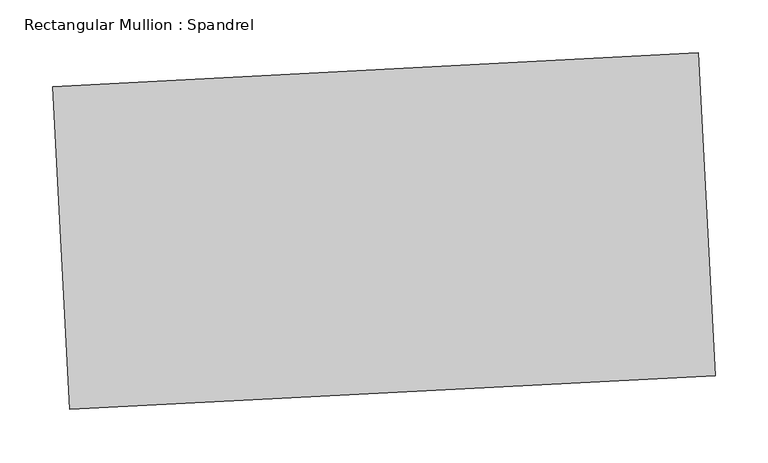
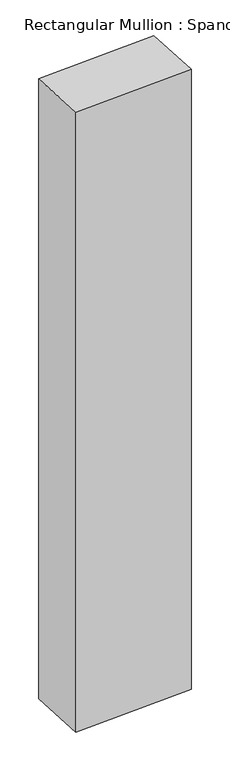
"""IFC4 building model written with IfcOpenShell, lengths in millimetres: member geometry, Rectangular Mullion : Spandrel."""

import ifcopenshell
import ifcopenshell.guid

model = None  # the IFC model being written
_history = None  # IfcOwnerHistory: only IFC2X3 demands one
_inside = {}  # id of a spatial element -> (the spatial element, [elements in it])
_under = {}  # id of a project, library or spatial element -> (it, [spatial elements below it])
_declared = {}  # id of a project -> (the project, [libraries it declares])
_typed = {}  # id of a type object -> (the type object, [elements of that type])
_made_of = {}  # id of a material, layer set ... -> (it, [elements and type objects made of it])


def new_model(schema):
    """Start an empty IFC model of exactly this schema.

    Asked for "IFC4X3", IfcOpenShell would pick the latest addendum, in which some entities
    have other attributes; the version numbers below select the first issue.
    IFC2X3 requires an IfcOwnerHistory on every rooted entity: one is made here for all.
    """
    global model, _history
    if schema == "IFC4X3":
        model = ifcopenshell.file(schema_version=(4, 3, 0, 0))
    else:
        model = ifcopenshell.file(schema=schema)
    _inside.clear()
    _under.clear()
    _declared.clear()
    _typed.clear()
    _made_of.clear()
    _history = None
    if model.schema == "IFC2X3":
        org = make("IfcOrganization", Name="unknown")
        user = make(
            "IfcPersonAndOrganization",
            ThePerson=make("IfcPerson", FamilyName="unknown"),
            TheOrganization=org,
        )
        app = make(
            "IfcApplication",
            ApplicationDeveloper=org,
            Version="unknown",
            ApplicationFullName="unknown",
            ApplicationIdentifier="unknown",
        )
        _history = make(
            "IfcOwnerHistory",
            OwningUser=user,
            OwningApplication=app,
            ChangeAction="ADDED",
            CreationDate=0,
        )
    return model


def make(cls, **values):
    """One entity of the class cls with the attributes given. An attribute that is None is left unset."""
    return model.create_entity(
        cls, **{name: value for name, value in values.items() if value is not None}
    )


def rooted(cls, **values):
    """An entity with a GlobalId (a new one), such as an element, a storey or a relation."""
    return make(cls, GlobalId=ifcopenshell.guid.new(), OwnerHistory=_history, **values)


def si_unit(unit_type, name, prefix=None):
    """IfcSIUnit, for example si_unit("LENGTHUNIT", "METRE", prefix="MILLI")."""
    return make("IfcSIUnit", UnitType=unit_type, Prefix=prefix, Name=name)


def assignment(units):
    """IfcUnitAssignment: the units of a project."""
    return None if units is None else make("IfcUnitAssignment", Units=units)


def point(xyz):
    """IfcCartesianPoint."""
    return None if xyz is None else make("IfcCartesianPoint", Coordinates=xyz)


def direction(xyz):
    """IfcDirection."""
    return None if xyz is None else make("IfcDirection", DirectionRatios=xyz)


def frame(location, z_axis=None, x_axis=None):
    """IfcAxis2Placement3D, a coordinate frame: its origin and axes. An axis left out is left unset."""
    return make(
        "IfcAxis2Placement3D",
        Location=point(location),
        Axis=direction(z_axis),
        RefDirection=direction(x_axis),
    )


def origin():
    """The frame at (0, 0, 0) with its axes left unset."""
    return frame((0.0, 0.0, 0.0))


def place(relative_to, where):
    """IfcLocalPlacement: puts the frame where relative to a parent placement (None: the world)."""
    return make(
        "IfcLocalPlacement", PlacementRelTo=relative_to, RelativePlacement=where
    )


def context(
    kind, dimensions, precision=None, world=None, true_north=None, identifier=None
):
    """IfcGeometricRepresentationContext, for example the 3D "Model" context."""
    return make(
        "IfcGeometricRepresentationContext",
        ContextIdentifier=identifier,
        ContextType=kind,
        CoordinateSpaceDimension=dimensions,
        Precision=precision,
        WorldCoordinateSystem=world,
        TrueNorth=true_north,
    )


def project(units=None, contexts=None):
    """IfcProject with its units and contexts."""
    return rooted(
        "IfcProject",
        Name="project",
        RepresentationContexts=contexts,
        UnitsInContext=assignment(units),
    )


def spatial(cls, under=None, at=None, **own):
    """A site, building, storey or space (cls), placed at a placement, below another one or the project."""
    s = rooted(cls, ObjectPlacement=at, **own)
    if under is not None:
        _under.setdefault(under.id(), (under, []))[1].append(s)
    return s


def polyline(points):
    """IfcPolyline through the points."""
    return make("IfcPolyline", Points=[point(p) for p in points])


def outline(outer, holes=None, kind="AREA"):
    """IfcArbitraryClosedProfileDef: a profile drawn as a closed curve; with holes, ...WithVoids."""
    if holes is None:
        return make("IfcArbitraryClosedProfileDef", ProfileType=kind, OuterCurve=outer)
    return make(
        "IfcArbitraryProfileDefWithVoids",
        ProfileType=kind,
        OuterCurve=outer,
        InnerCurves=holes,
    )


def extrude(swept, where, along, depth):
    """IfcExtrudedAreaSolid: the profile swept, set in the frame where, extruded along a direction by depth."""
    return make(
        "IfcExtrudedAreaSolid",
        SweptArea=swept,
        Position=where,
        ExtrudedDirection=direction(along),
        Depth=depth,
    )


def shape(context_of_items, identifier, shape_type, items):
    """IfcShapeRepresentation: the items that make up one representation, for example the "Body"."""
    return make(
        "IfcShapeRepresentation",
        ContextOfItems=context_of_items,
        RepresentationIdentifier=identifier,
        RepresentationType=shape_type,
        Items=items,
    )


def source(mapping_origin, context_of_items, identifier, shape_type, items):
    """IfcRepresentationMap: a shape defined once, which mapped items show again and again."""
    return make(
        "IfcRepresentationMap",
        MappingOrigin=mapping_origin,
        MappedRepresentation=shape(context_of_items, identifier, shape_type, items),
    )


def transform(
    local_origin,
    x_axis=None,
    y_axis=None,
    z_axis=None,
    scale=None,
    scale2=None,
    scale3=None,
    uniform=True,
):
    """IfcCartesianTransformationOperator3D, or its non-uniform kind. x_axis, y_axis, z_axis: its Axis1, 2, 3."""
    if uniform:
        return make(
            "IfcCartesianTransformationOperator3D",
            Axis1=direction(x_axis),
            Axis2=direction(y_axis),
            LocalOrigin=point(local_origin),
            Scale=scale,
            Axis3=direction(z_axis),
        )
    return make(
        "IfcCartesianTransformationOperator3DnonUniform",
        Axis1=direction(x_axis),
        Axis2=direction(y_axis),
        LocalOrigin=point(local_origin),
        Scale=scale,
        Axis3=direction(z_axis),
        Scale2=scale2,
        Scale3=scale3,
    )


def mapped(mapping_source, mapping_target):
    """IfcMappedItem: shows the shape of a source again, moved by a transform."""
    return make(
        "IfcMappedItem", MappingSource=mapping_source, MappingTarget=mapping_target
    )


def made_of(thing, what):
    """Note that an element or type object is made of a material, layer set ...; save() writes the relation."""
    if what is not None:
        _made_of.setdefault(what.id(), (what, []))[1].append(thing)
    return thing


def element(
    cls,
    number,
    at=None,
    inside=None,
    cuts=None,
    type_object=None,
    material=None,
    context=None,
    identifier="Body",
    shape_type=None,
    held_by="IfcProductDefinitionShape",
    body=None,
    shapes=None,
    **own,
):
    """One element of the class cls, such as IfcWall. Its Tag is "e" and its number.

    at: its placement. inside: the storey or other place that contains it. cuts: it is an
    opening in that element (IfcRelVoidsElement). A single representation is given by context,
    identifier, shape_type and body (its items); several are given by shapes. held_by: the class
    of the entity that holds the representations. save() writes the other relations.
    """
    e = rooted(cls, Tag="e%d" % number, ObjectPlacement=at, **own)
    if body is not None:
        shapes = [shape(context, identifier, shape_type, body)]
    if shapes is not None:
        e.Representation = make(held_by, Representations=shapes)
    if inside is not None:
        _inside.setdefault(inside.id(), (inside, []))[1].append(e)
    if cuts is not None:
        rooted(
            "IfcRelVoidsElement", RelatingBuildingElement=cuts, RelatedOpeningElement=e
        )
    if type_object is not None:
        _typed.setdefault(type_object.id(), (type_object, []))[1].append(e)
    return made_of(e, material)


def aggregate(whole, parts):
    """IfcRelAggregates: a whole, such as a stair, and the parts it consists of."""
    return rooted("IfcRelAggregates", RelatingObject=whole, RelatedObjects=parts)


def save(model, path):
    """Write the relations noted so far, then the file.

    IfcRelAggregates (storeys below a building ...), IfcRelContainedInSpatialStructure (elements
    in a storey), IfcRelDefinesByType, IfcRelAssociatesMaterial and IfcRelDeclares: one each for
    every whole, place, type object, material and project.
    """
    for whole, parts in _under.values():
        aggregate(whole, parts)
    for where, things in _inside.values():
        rooted(
            "IfcRelContainedInSpatialStructure",
            RelatedElements=things,
            RelatingStructure=where,
        )
    for kind, things in _typed.values():
        rooted("IfcRelDefinesByType", RelatedObjects=things, RelatingType=kind)
    for what, things in _made_of.values():
        rooted("IfcRelAssociatesMaterial", RelatedObjects=things, RelatingMaterial=what)
    for by, libraries in _declared.values():
        rooted("IfcRelDeclares", RelatingContext=by, RelatedDefinitions=libraries)
    model.write(path)


def rectangular_mullion_spandrel_3b5c7c06(model_context):
    return source(origin(), model_context, "Body", "SweptSolid", [
        extrude(outline(polyline([(-617.1582819, 136.2391416), (-8.3937175, 168.1431406), (7.5582819, -136.2391416), (-601.2062825, -168.1431406), (-617.1582819, 136.2391416)])), frame((0.0, 0.0, -3352.8), z_axis=(0.0, 0.0, 1.0), x_axis=(1.0, 0.0, 0.0)), (0.0, 0.0, 1.0), 3352.8),
    ])


if __name__ == "__main__":
    model = new_model("IFC4")
    model_context = context("Model", 3, world=origin())
    ifc_project = project(units=[si_unit("LENGTHUNIT", "METRE", prefix="MILLI")], contexts=[model_context])
    site = spatial("IfcSite", under=ifc_project)
    building = spatial("IfcBuilding", under=site)
    placement = place(None, origin())
    rectangular_mullion_spandrel_shape = rectangular_mullion_spandrel_3b5c7c06(model_context)
    element("IfcMember", 1, ObjectType="Rectangular Mullion : Spandrel", at=placement, inside=building, context=model_context, shape_type="MappedRepresentation", body=[
        mapped(rectangular_mullion_spandrel_shape, transform((0.0, 0.0, 0.0), x_axis=(1.0, 0.0, 0.0), y_axis=(0.0, 1.0, 0.0), z_axis=(0.0, 0.0, 1.0))),
    ])
    save(model, "model.ifc")

# Revit data of these elements
# Project information
#   Organization Name = "G3B Press"
#   Organization Description = "Paul F. Aubin Cosulting Services, Inc."
#   Building Name = "Revit Essentials for Architecture"
#   Author = "Paul F. Aubin"
#   Author Website = "https://www.paulaubin.com"
#   Copyright = "Copyright © 2020 Paul F Aubin, all rights reserved"
#   Design Option = "Main Model"
#   Project Issue Date = "8/1/2020"
#   Project Status = "Design Development"
#   Client Name = "Families and the Family Editor"
#   Project Address = "123 State ST\nSuite 301\nChicago, IL 60606"
#   Project Name = "11 Commercial_Complete"
#   Project Number = "2020.04A"
# Type "Rectangular Mullion : Spandrel"
#   built-in parameter 1007304 = 1 (stored number, unit not read)
#   built-in parameter 1007301 = 1 (stored number, unit not read)
#   built-in parameter 1007300 = 1 (stored number, unit not read)
# Element 1 (IfcMember, "Rectangular Mullion : Spandrel")
#   Materials on its faces: "Aluminum"
# Materials
#   "Aluminum": class "Metal", colour RGB 247 247 247, transparency 0, Description = "Aluminum 6061", Cost = 0
